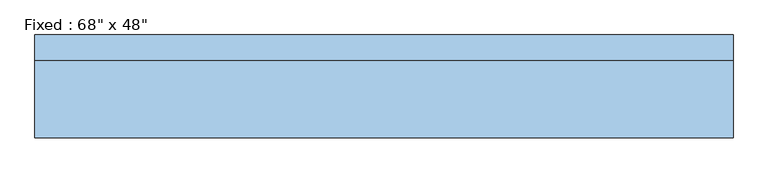
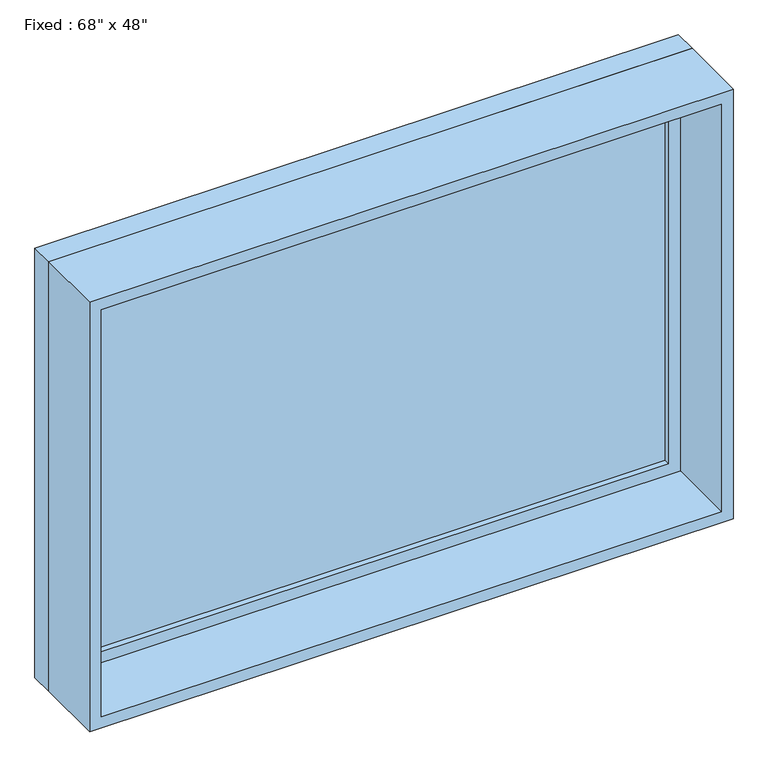
"""IFC4 building model written with IfcOpenShell, lengths in millimetres: window geometry."""

from ifc_helpers import new_model, si_unit, frame, origin, place, context, project, spatial, polyline, outline, extrude, source, transform, mapped, element, save


def window_01d19bfd(model_context):
    return source(origin(), model_context, "Body", "SweptSolid", [
        extrude(outline(polyline([(762.0, 79.375), (-838.2, 79.375), (-838.2, 92.075), (762.0, 92.075), (762.0, 79.375)])), frame((0.0, 0.0, 368.3), z_axis=(0.0, 0.0, 1.0), x_axis=(1.0, 0.0, 0.0)), (0.0, 0.0, 1.0), 1092.2),
        extrude(outline(polyline([(1504.95, -882.65), (323.85, -882.65), (323.85, 806.45), (1504.95, 806.45), (1504.95, -882.65)]), holes=[polyline([(1460.5, -838.2), (1460.5, 762.0), (368.3, 762.0), (368.3, -838.2), (1460.5, -838.2)])]), frame((0.0, 63.5, 0.0), z_axis=(0.0, 1.0, 0.0), x_axis=(0.0, 0.0, 1.0)), (0.0, 0.0, 1.0), 44.45),
        extrude(outline(polyline([(1524.0, -901.7), (304.8, -901.7), (304.8, 825.5), (1524.0, 825.5), (1524.0, -901.7)]), holes=[polyline([(1492.25, -869.95), (1492.25, 793.75), (336.55, 793.75), (336.55, -869.95), (1492.25, -869.95)])]), frame((0.0, -127.0, 0.0), z_axis=(0.0, 1.0, 0.0), x_axis=(0.0, 0.0, 1.0)), (0.0, 0.0, 1.0), 190.5),
        extrude(outline(polyline([(1524.0, 825.5), (1524.0, -901.7), (304.8, -901.7), (304.8, 825.5), (1524.0, 825.5)]), holes=[polyline([(1504.95, 806.45), (323.85, 806.45), (323.85, -882.65), (1504.95, -882.65), (1504.95, 806.45)])]), frame((0.0, 63.5, 0.0), z_axis=(0.0, 1.0, 0.0), x_axis=(0.0, 0.0, 1.0)), (0.0, 0.0, 1.0), 63.5),
    ])


if __name__ == "__main__":
    model = new_model("IFC4")
    model_context = context("Model", 3, world=origin())
    ifc_project = project(units=[si_unit("LENGTHUNIT", "METRE", prefix="MILLI")], contexts=[model_context])
    site = spatial("IfcSite", under=ifc_project)
    building = spatial("IfcBuilding", under=site)
    placement = place(None, origin())
    window_shape = window_01d19bfd(model_context)
    element("IfcWindow", 1, ObjectType="Fixed : 68\" x 48\"", at=placement, inside=building, context=model_context, shape_type="MappedRepresentation", body=[
        mapped(window_shape, transform((0.0, 0.0, 0.0), x_axis=(1.0, 0.0, 0.0), y_axis=(0.0, 1.0, 0.0), z_axis=(0.0, 0.0, 1.0))),
    ])
    save(model, "model.ifc")

# Revit data of these elements
# Type "Fixed : 68\" x 48\""
#   Type Mark = "17"
#   Assembly Code = "B2020100"
#   Height = 1219.2 mm
#   Default Sill Height = 304.8 mm
#   Width = 1727.2 mm
#   Window Inset = 19.05 mm
#   Glass Pane Material = Glass
#   Sash Material = Sash
#   Wall Closure = (empty or 0)
# Element 1 (IfcWindow, "Fixed : 68\" x 48\"")
#   Materials on its faces: "Sash", "Glass"
# Materials
#   "Glass": class "Glass", colour RGB 0 128 192, transparency 0.75
#   "Sash": class "Wood", colour RGB 224 178 126, transparency 0
